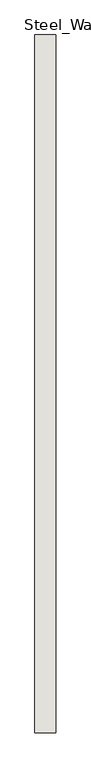
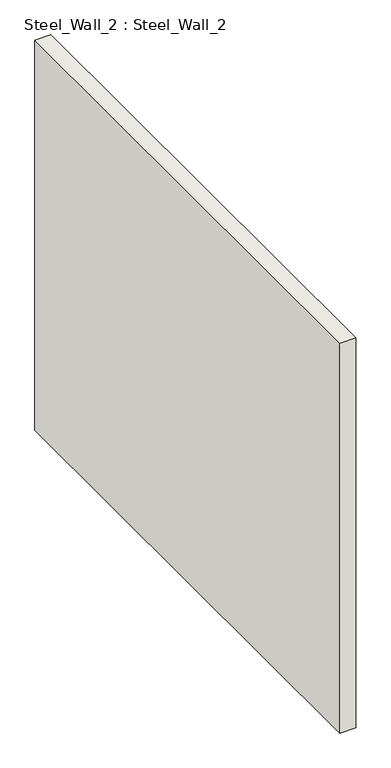
"""IFC4 building model written with IfcOpenShell, lengths in millimetres: wall geometry, Steel_Wall_2 : Steel_Wall_2."""

from ifc_helpers import new_model, si_unit, frame, origin, place, context, project, spatial, polyline, outline, extrude, source, transform, mapped, element, save


def steel_wall_2_steel_wall_2_9d9e34b6(model_context):
    return source(origin(), model_context, "Body", "SweptSolid", [
        extrude(outline(polyline([(215.0, 7495.0), (215.0, 4165.0), (115.0, 4165.0), (115.0, 7495.0), (215.0, 7495.0)])), frame((0.0, 0.0, 250.0), z_axis=(0.0, 0.0, 1.0), x_axis=(1.0, 0.0, 0.0)), (0.0, 0.0, 1.0), 2600.0),
    ])


if __name__ == "__main__":
    model = new_model("IFC4")
    model_context = context("Model", 3, world=origin())
    ifc_project = project(units=[si_unit("LENGTHUNIT", "METRE", prefix="MILLI")], contexts=[model_context])
    site = spatial("IfcSite", under=ifc_project)
    building = spatial("IfcBuilding", under=site)
    placement = place(None, origin())
    steel_wall_2_steel_wall_2_shape = steel_wall_2_steel_wall_2_9d9e34b6(model_context)
    element("IfcWall", 1, ObjectType="Steel_Wall_2 : Steel_Wall_2", at=placement, inside=building, context=model_context, shape_type="MappedRepresentation", body=[
        mapped(steel_wall_2_steel_wall_2_shape, transform((0.0, 0.0, 0.0), x_axis=(1.0, 0.0, 0.0), y_axis=(0.0, 1.0, 0.0), z_axis=(0.0, 0.0, 1.0))),
    ])
    save(model, "model.ifc")

# Revit data of these elements
# Type "Steel_Wall_2 : Steel_Wall_2"
#   NameOverride = "Steel_Wall_2"
# Element 1 (IfcWall, "Steel_Wall_2 : Steel_Wall_2")
#   Materials on its faces: "IfcSurfaceStyle #33"
# Materials
#   "IfcSurfaceStyle #33": class "Unassigned", colour RGB 214 214 214, transparency 0
